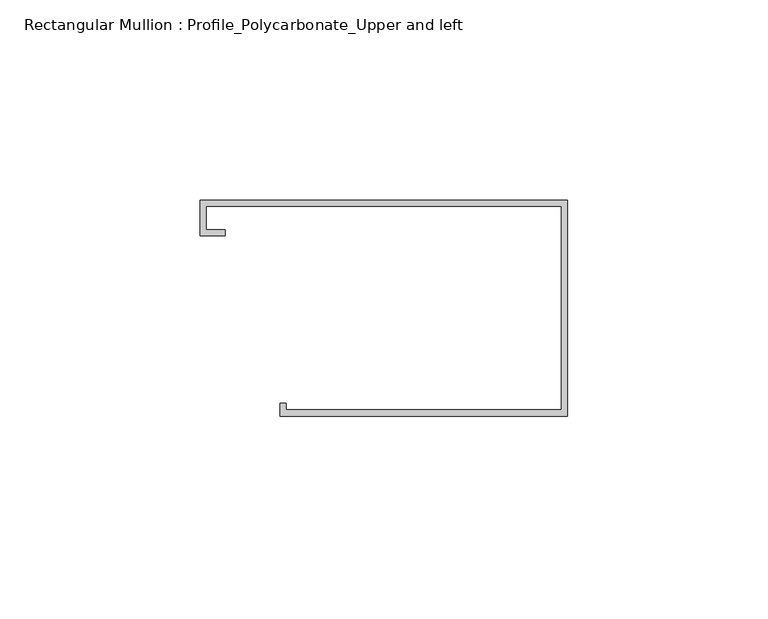
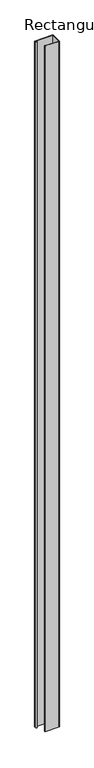
"""IFC4 building model written with IfcOpenShell, lengths in millimetres: member geometry, Rectangular Mullion : Profile_Polycarbonate_Upper and left."""

from ifc_helpers import new_model, si_unit, frame, origin, place, context, project, spatial, polyline, outline, extrude, source, transform, mapped, element, save


def rectangular_mullion_profile_polycarbonate_upper_and_left_db2f125b(model_context):
    return source(origin(), model_context, "Body", "SweptSolid", [
        extrude(outline(polyline([(0.0, 28.984575), (0.0, -25.015825), (-71.9836, -25.015825), (-71.9836, -21.840825), (-70.3961, -21.840825), (-70.3961, -23.428325), (-1.5875, -23.428325), (-1.5875, 27.397075), (-90.4113, 27.397075), (-90.4113, 21.580475), (-85.6488, 21.580475), (-85.6488, 19.992975), (-91.9988, 19.992975), (-91.9988, 28.984575), (0.0, 28.984575)])), frame((0.0, 0.0, -3622.5713735), z_axis=(0.0, 0.0, 1.0), x_axis=(1.0, 0.0, 0.0)), (0.0, 0.0, 1.0), 3622.5713735),
    ])


if __name__ == "__main__":
    model = new_model("IFC4")
    model_context = context("Model", 3, world=origin())
    ifc_project = project(units=[si_unit("LENGTHUNIT", "METRE", prefix="MILLI")], contexts=[model_context])
    site = spatial("IfcSite", under=ifc_project)
    building = spatial("IfcBuilding", under=site)
    placement = place(None, origin())
    rectangular_mullion_profile_polycarbonate_upper_and_left_shape = rectangular_mullion_profile_polycarbonate_upper_and_left_db2f125b(model_context)
    element("IfcMember", 1, ObjectType="Rectangular Mullion : Profile_Polycarbonate_Upper and left", at=placement, inside=building, context=model_context, shape_type="MappedRepresentation", body=[
        mapped(rectangular_mullion_profile_polycarbonate_upper_and_left_shape, transform((0.0, 0.0, 0.0), x_axis=(1.0, 0.0, 0.0), y_axis=(0.0, 1.0, 0.0), z_axis=(0.0, 0.0, 1.0))),
    ])
    save(model, "model.ifc")

# Revit data of these elements
# Type "Rectangular Mullion : Profile_Polycarbonate_Upper and left"
#   built-in parameter 1007322 = 0.177167 (stored number, unit not read)
#   built-in parameter 1007321 = 0.00520833 (stored number, unit not read)
#   built-in parameter 1007320 = 0 (stored number, unit not read)
